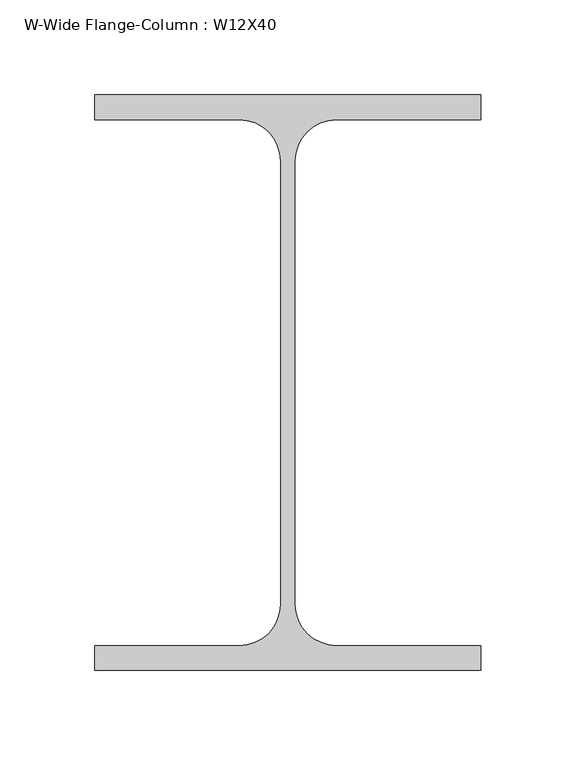
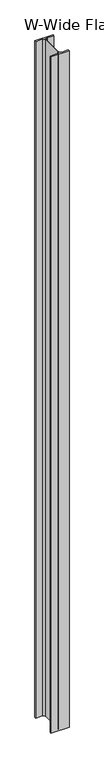
"""IFC4 building model written with IfcOpenShell, lengths in millimetres: column geometry, W-Wide Flange-Column : W12X40."""

from ifc_helpers import new_model, si_unit, point, frame, frame_2d, origin, place, context, project, spatial, polyline, circle_curve, trimmed, segment, composite_curve, outline, extrude, source, transform, mapped, element, save


def w_wide_flange_column_w12x40_bfea6e2c(model_context):
    return source(origin(), model_context, "Body", "SweptSolid", [
        extrude(outline(composite_curve([segment(polyline([(101.6496094, 151.6558594), (101.6496094, 138.5589844), (25.5984375, 138.5589844)]), True, "CONTINUOUS"), segment(trimmed(circle_curve(frame_2d((25.5984375, 116.7308594)), 21.828125), [point((25.5984375, 138.5589844))], [point((3.7703125, 116.7308594))], True, "CARTESIAN"), True, "CONTINUOUS"), segment(polyline([(3.7703125, 116.7308594), (3.7703125, -116.7308594)]), True, "CONTINUOUS"), segment(trimmed(circle_curve(frame_2d((25.5984375, -116.7308594)), 21.828125), [point((3.7703125, -116.7308594))], [point((25.5984375, -138.5589844))], True, "CARTESIAN"), True, "CONTINUOUS"), segment(polyline([(25.5984375, -138.5589844), (101.6496094, -138.5589844), (101.6496094, -151.6558594), (-101.6496094, -151.6558594), (-101.6496094, -138.5589844), (-25.5984375, -138.5589844)]), True, "CONTINUOUS"), segment(trimmed(circle_curve(frame_2d((-25.5984375, -116.7308594)), 21.828125), [point((-25.5984375, -138.5589844))], [point((-3.7703125, -116.7308594))], True, "CARTESIAN"), True, "CONTINUOUS"), segment(polyline([(-3.7703125, -116.7308594), (-3.7703125, 116.7308594)]), True, "CONTINUOUS"), segment(trimmed(circle_curve(frame_2d((-25.5984375, 116.7308594)), 21.828125), [point((-3.7703125, 116.7308594))], [point((-25.5984375, 138.5589844))], True, "CARTESIAN"), True, "CONTINUOUS"), segment(polyline([(-25.5984375, 138.5589844), (-101.6496094, 138.5589844), (-101.6496094, 151.6558594), (101.6496094, 151.6558594)]), True, "CONTINUOUS")], self_intersect=False)), frame((0.0, 0.0, 30480.0), z_axis=(0.0, 0.0, 1.0), x_axis=(1.0, 0.0, 0.0)), (0.0, 0.0, 1.0), 7924.8),
    ])


if __name__ == "__main__":
    model = new_model("IFC4")
    model_context = context("Model", 3, world=origin())
    ifc_project = project(units=[si_unit("LENGTHUNIT", "METRE", prefix="MILLI")], contexts=[model_context])
    site = spatial("IfcSite", under=ifc_project)
    building = spatial("IfcBuilding", under=site)
    placement = place(None, origin())
    w_wide_flange_column_w12x40_shape = w_wide_flange_column_w12x40_bfea6e2c(model_context)
    element("IfcColumn", 1, ObjectType="W-Wide Flange-Column : W12X40", at=placement, inside=building, context=model_context, shape_type="MappedRepresentation", body=[
        mapped(w_wide_flange_column_w12x40_shape, transform((0.0, 0.0, 0.0), x_axis=(1.0, 0.0, 0.0), y_axis=(0.0, 1.0, 0.0), z_axis=(0.0, 0.0, 1.0))),
    ])
    save(model, "model.ifc")

# Revit data of these elements
# Type "W-Wide Flange-Column : W12X40"
#   Assembly Code = "B10"
#   W = 40
#   bf = 203.299 mm
#   d = 303.312 mm
#   k = 34.925 mm
#   kr = 21.828 mm
#   tf = 13.097 mm
#   tw = 7.541 mm
#   A = 0.00761289 m²
#   Structural Material [instance default] = Steel ASTM A992
# Element 1 (IfcColumn, "W-Wide Flange-Column : W12X40")
#   Structural Material = Aluminum, Anodized Red
#   Materials on its faces: "Aluminum, Anodized Red"
# Materials
#   "Steel ASTM A992": class "Metal", colour RGB 128 0 0, transparency 0, Description = "Structural steel 50ksi", Cost = 0
#   "Aluminum, Anodized Red": class "Metal", colour RGB 120 120 120, transparency 0, Description = "Anodized aluminum, red", Cost = 0
